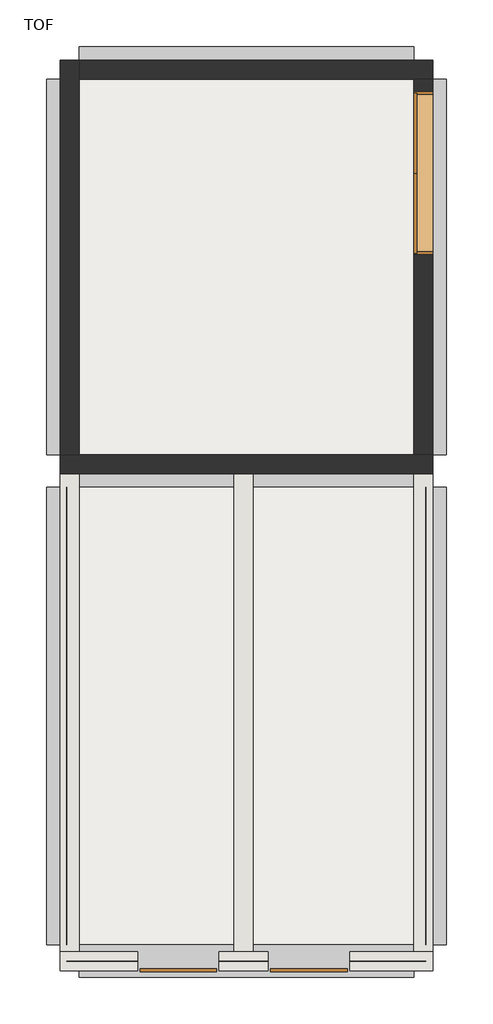
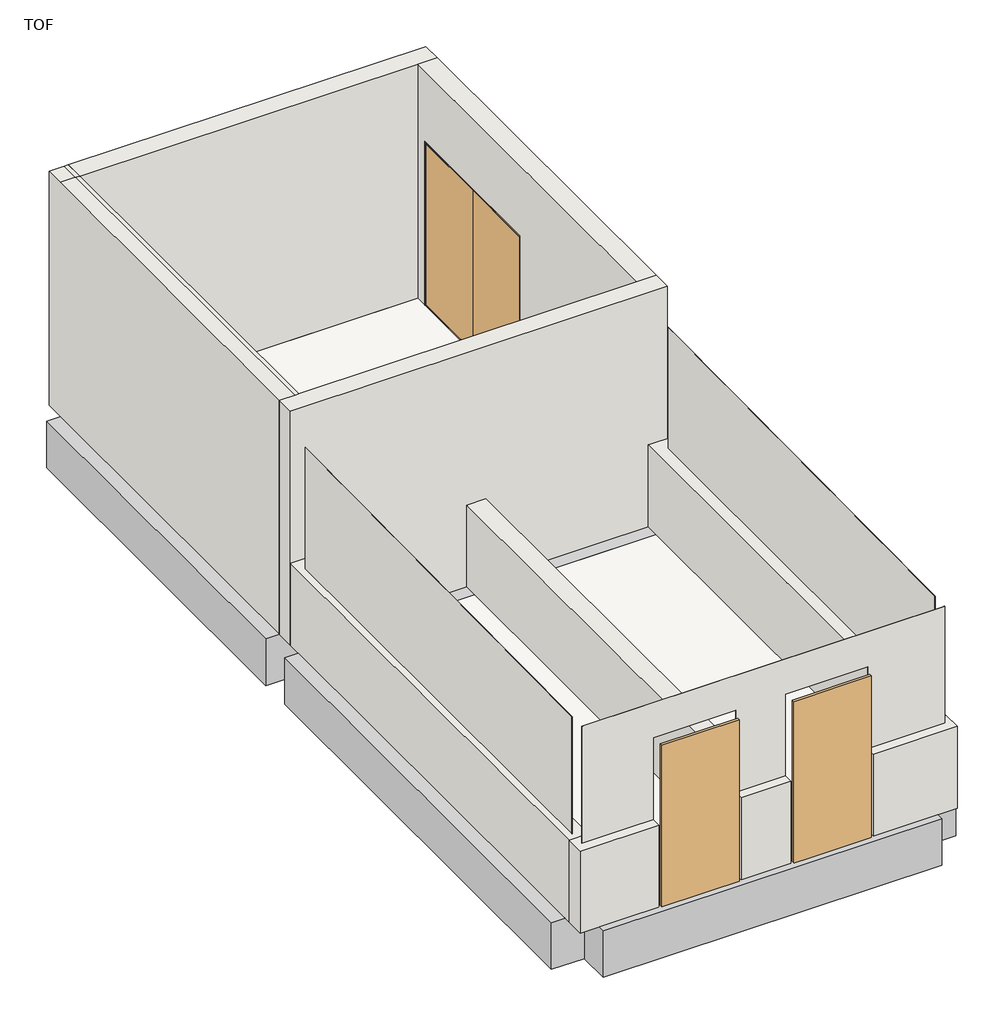
# One storey: 11 walls, 7 beams, 3 doors, 2 slabs.
"""IFC4 building model written with IfcOpenShell, lengths in millimetres."""

import ifcopenshell
import ifcopenshell.guid

model = None  # the IFC model being written
_history = None  # IfcOwnerHistory: only IFC2X3 demands one
_inside = {}  # id of a spatial element -> (the spatial element, [elements in it])
_under = {}  # id of a project, library or spatial element -> (it, [spatial elements below it])
_declared = {}  # id of a project -> (the project, [libraries it declares])
_typed = {}  # id of a type object -> (the type object, [elements of that type])
_made_of = {}  # id of a material, layer set ... -> (it, [elements and type objects made of it])


def new_model(schema):
    """Start an empty IFC model of exactly this schema.

    Asked for "IFC4X3", IfcOpenShell would pick the latest addendum, in which some entities
    have other attributes; the version numbers below select the first issue.
    IFC2X3 requires an IfcOwnerHistory on every rooted entity: one is made here for all.
    """
    global model, _history
    if schema == "IFC4X3":
        model = ifcopenshell.file(schema_version=(4, 3, 0, 0))
    else:
        model = ifcopenshell.file(schema=schema)
    _inside.clear()
    _under.clear()
    _declared.clear()
    _typed.clear()
    _made_of.clear()
    _history = None
    if model.schema == "IFC2X3":
        org = make("IfcOrganization", Name="unknown")
        user = make(
            "IfcPersonAndOrganization",
            ThePerson=make("IfcPerson", FamilyName="unknown"),
            TheOrganization=org,
        )
        app = make(
            "IfcApplication",
            ApplicationDeveloper=org,
            Version="unknown",
            ApplicationFullName="unknown",
            ApplicationIdentifier="unknown",
        )
        _history = make(
            "IfcOwnerHistory",
            OwningUser=user,
            OwningApplication=app,
            ChangeAction="ADDED",
            CreationDate=0,
        )
    return model


def make(cls, **values):
    """One entity of the class cls with the attributes given. An attribute that is None is left unset."""
    return model.create_entity(
        cls, **{name: value for name, value in values.items() if value is not None}
    )


def rooted(cls, **values):
    """An entity with a GlobalId (a new one), such as an element, a storey or a relation."""
    return make(cls, GlobalId=ifcopenshell.guid.new(), OwnerHistory=_history, **values)


def si_unit(unit_type, name, prefix=None):
    """IfcSIUnit, for example si_unit("LENGTHUNIT", "METRE", prefix="MILLI")."""
    return make("IfcSIUnit", UnitType=unit_type, Prefix=prefix, Name=name)


def assignment(units):
    """IfcUnitAssignment: the units of a project."""
    return None if units is None else make("IfcUnitAssignment", Units=units)


def point(xyz):
    """IfcCartesianPoint."""
    return None if xyz is None else make("IfcCartesianPoint", Coordinates=xyz)


def direction(xyz):
    """IfcDirection."""
    return None if xyz is None else make("IfcDirection", DirectionRatios=xyz)


def frame(location, z_axis=None, x_axis=None):
    """IfcAxis2Placement3D, a coordinate frame: its origin and axes. An axis left out is left unset."""
    return make(
        "IfcAxis2Placement3D",
        Location=point(location),
        Axis=direction(z_axis),
        RefDirection=direction(x_axis),
    )


def origin():
    """The frame at (0, 0, 0) with its axes left unset."""
    return frame((0.0, 0.0, 0.0))


def origin_with_axes():
    """The frame at (0, 0, 0) with the z axis (0, 0, 1) and the x axis (1, 0, 0) written out."""
    return frame((0.0, 0.0, 0.0), z_axis=(0.0, 0.0, 1.0), x_axis=(1.0, 0.0, 0.0))


def place(relative_to, where):
    """IfcLocalPlacement: puts the frame where relative to a parent placement (None: the world)."""
    return make(
        "IfcLocalPlacement", PlacementRelTo=relative_to, RelativePlacement=where
    )


def context(
    kind, dimensions, precision=None, world=None, true_north=None, identifier=None
):
    """IfcGeometricRepresentationContext, for example the 3D "Model" context."""
    return make(
        "IfcGeometricRepresentationContext",
        ContextIdentifier=identifier,
        ContextType=kind,
        CoordinateSpaceDimension=dimensions,
        Precision=precision,
        WorldCoordinateSystem=world,
        TrueNorth=true_north,
    )


def project(units=None, contexts=None):
    """IfcProject with its units and contexts."""
    return rooted(
        "IfcProject",
        Name="project",
        RepresentationContexts=contexts,
        UnitsInContext=assignment(units),
    )


def spatial(cls, under=None, at=None, **own):
    """A site, building, storey or space (cls), placed at a placement, below another one or the project."""
    s = rooted(cls, ObjectPlacement=at, **own)
    if under is not None:
        _under.setdefault(under.id(), (under, []))[1].append(s)
    return s


def polyline(points):
    """IfcPolyline through the points."""
    return make("IfcPolyline", Points=[point(p) for p in points])


def outline(outer, holes=None, kind="AREA"):
    """IfcArbitraryClosedProfileDef: a profile drawn as a closed curve; with holes, ...WithVoids."""
    if holes is None:
        return make("IfcArbitraryClosedProfileDef", ProfileType=kind, OuterCurve=outer)
    return make(
        "IfcArbitraryProfileDefWithVoids",
        ProfileType=kind,
        OuterCurve=outer,
        InnerCurves=holes,
    )


def extrude(swept, where, along, depth):
    """IfcExtrudedAreaSolid: the profile swept, set in the frame where, extruded along a direction by depth."""
    return make(
        "IfcExtrudedAreaSolid",
        SweptArea=swept,
        Position=where,
        ExtrudedDirection=direction(along),
        Depth=depth,
    )


def faces_of(points, faces, orient=None, outer=None):
    """IfcFace entities. A face is a list of loops; a loop is a list of indices into points, from 0.

    orient and outer hold one flag for each loop. By default every Orientation is true, the
    first loop of a face is its IfcFaceOuterBound and the others are IfcFaceBound.
    """
    made = []
    for i, loops in enumerate(faces):
        bounds = []
        for j, loop in enumerate(loops):
            is_outer = j == 0 if outer is None else outer[i][j]
            bounds.append(
                make(
                    "IfcFaceOuterBound" if is_outer else "IfcFaceBound",
                    Bound=make("IfcPolyLoop", Polygon=[points[k] for k in loop]),
                    Orientation=True if orient is None else orient[i][j],
                )
            )
        made.append(make("IfcFace", Bounds=bounds))
    return made


def faceted_brep(points, faces, orient=None, outer=None, voids=None):
    """IfcFacetedBrep: a solid bounded by flat faces; with voids (closed shells), ...WithVoids."""
    shared = [point(p) for p in points]
    hull = make("IfcClosedShell", CfsFaces=faces_of(shared, faces, orient, outer))
    if voids is None:
        return make("IfcFacetedBrep", Outer=hull)
    return make(
        "IfcFacetedBrepWithVoids",
        Outer=hull,
        Voids=[
            make(cls, CfsFaces=faces_of(shared, fs, o, b)) for cls, fs, o, b in voids
        ],
    )


def shape(context_of_items, identifier, shape_type, items):
    """IfcShapeRepresentation: the items that make up one representation, for example the "Body"."""
    return make(
        "IfcShapeRepresentation",
        ContextOfItems=context_of_items,
        RepresentationIdentifier=identifier,
        RepresentationType=shape_type,
        Items=items,
    )


def source(mapping_origin, context_of_items, identifier, shape_type, items):
    """IfcRepresentationMap: a shape defined once, which mapped items show again and again."""
    return make(
        "IfcRepresentationMap",
        MappingOrigin=mapping_origin,
        MappedRepresentation=shape(context_of_items, identifier, shape_type, items),
    )


def transform(
    local_origin,
    x_axis=None,
    y_axis=None,
    z_axis=None,
    scale=None,
    scale2=None,
    scale3=None,
    uniform=True,
):
    """IfcCartesianTransformationOperator3D, or its non-uniform kind. x_axis, y_axis, z_axis: its Axis1, 2, 3."""
    if uniform:
        return make(
            "IfcCartesianTransformationOperator3D",
            Axis1=direction(x_axis),
            Axis2=direction(y_axis),
            LocalOrigin=point(local_origin),
            Scale=scale,
            Axis3=direction(z_axis),
        )
    return make(
        "IfcCartesianTransformationOperator3DnonUniform",
        Axis1=direction(x_axis),
        Axis2=direction(y_axis),
        LocalOrigin=point(local_origin),
        Scale=scale,
        Axis3=direction(z_axis),
        Scale2=scale2,
        Scale3=scale3,
    )


def mapped(mapping_source, mapping_target):
    """IfcMappedItem: shows the shape of a source again, moved by a transform."""
    return make(
        "IfcMappedItem", MappingSource=mapping_source, MappingTarget=mapping_target
    )


def made_of(thing, what):
    """Note that an element or type object is made of a material, layer set ...; save() writes the relation."""
    if what is not None:
        _made_of.setdefault(what.id(), (what, []))[1].append(thing)
    return thing


def element(
    cls,
    number,
    at=None,
    inside=None,
    cuts=None,
    type_object=None,
    material=None,
    context=None,
    identifier="Body",
    shape_type=None,
    held_by="IfcProductDefinitionShape",
    body=None,
    shapes=None,
    **own,
):
    """One element of the class cls, such as IfcWall. Its Tag is "e" and its number.

    at: its placement. inside: the storey or other place that contains it. cuts: it is an
    opening in that element (IfcRelVoidsElement). A single representation is given by context,
    identifier, shape_type and body (its items); several are given by shapes. held_by: the class
    of the entity that holds the representations. save() writes the other relations.
    """
    e = rooted(cls, Tag="e%d" % number, ObjectPlacement=at, **own)
    if body is not None:
        shapes = [shape(context, identifier, shape_type, body)]
    if shapes is not None:
        e.Representation = make(held_by, Representations=shapes)
    if inside is not None:
        _inside.setdefault(inside.id(), (inside, []))[1].append(e)
    if cuts is not None:
        rooted(
            "IfcRelVoidsElement", RelatingBuildingElement=cuts, RelatedOpeningElement=e
        )
    if type_object is not None:
        _typed.setdefault(type_object.id(), (type_object, []))[1].append(e)
    return made_of(e, material)


def aggregate(whole, parts):
    """IfcRelAggregates: a whole, such as a stair, and the parts it consists of."""
    return rooted("IfcRelAggregates", RelatingObject=whole, RelatedObjects=parts)


def save(model, path):
    """Write the relations noted so far, then the file.

    IfcRelAggregates (storeys below a building ...), IfcRelContainedInSpatialStructure (elements
    in a storey), IfcRelDefinesByType, IfcRelAssociatesMaterial and IfcRelDeclares: one each for
    every whole, place, type object, material and project.
    """
    for whole, parts in _under.values():
        aggregate(whole, parts)
    for where, things in _inside.values():
        rooted(
            "IfcRelContainedInSpatialStructure",
            RelatedElements=things,
            RelatingStructure=where,
        )
    for kind, things in _typed.values():
        rooted("IfcRelDefinesByType", RelatedObjects=things, RelatingType=kind)
    for what, things in _made_of.values():
        rooted("IfcRelAssociatesMaterial", RelatedObjects=things, RelatingMaterial=what)
    for by, libraries in _declared.values():
        rooted("IfcRelDeclares", RelatingContext=by, RelatedDefinitions=libraries)
    model.write(path)


def double_door_steel_cbf312ec(model_context):
    return source(origin(), model_context, "Body", "SolidModel", [
        extrude(outline(polyline([(980.0, 77.0), (0.0, 77.0), (0.0, 117.0), (980.0, 117.0), (980.0, 77.0)])), frame((0.0, 0.0, 20.0), z_axis=(0.0, 0.0, 1.0), x_axis=(1.0, 0.0, 0.0)), (0.0, 0.0, 1.0), 2060.0),
        extrude(outline(polyline([(0.0, 77.0), (-980.0, 77.0), (-980.0, 117.0), (0.0, 117.0), (0.0, 77.0)])), frame((0.0, 0.0, 20.0), z_axis=(0.0, 0.0, 1.0), x_axis=(1.0, 0.0, 0.0)), (0.0, 0.0, 1.0), 2060.0),
        faceted_brep([(1000.0, -117.0, 2100.0), (1000.0, 117.0, 2100.0), (-1000.0, 117.0, 2100.0), (-1000.0, -117.0, 2100.0), (965.0, 77.0, 2065.0), (965.0, -117.0, 2065.0), (-965.0, -117.0, 2065.0), (-965.0, 77.0, 2065.0), (980.0, 117.0, 2080.0), (980.0, 77.0, 2080.0), (-980.0, 77.0, 2080.0), (-980.0, 117.0, 2080.0), (-1000.0, 117.0, 0.0), (-1000.0, -117.0, 0.0), (-965.0, -117.0, 35.0), (-965.0, 77.0, 35.0), (-980.0, 77.0, 20.0), (-980.0, 117.0, 20.0), (1000.0, 117.0, 0.0), (980.0, 117.0, 20.0), (1000.0, -117.0, 0.0), (965.0, -117.0, 35.0), (965.0, 77.0, 35.0), (980.0, 77.0, 20.0)], [[[0, 1, 2, 3]], [[4, 5, 6, 7]], [[8, 9, 10, 11]], [[3, 2, 12, 13]], [[7, 6, 14, 15]], [[11, 10, 16, 17]], [[18, 12, 2, 1], [8, 11, 17, 19]], [[13, 12, 18, 20]], [[0, 3, 13, 20], [21, 14, 6, 5]], [[15, 14, 21, 22]], [[23, 16, 10, 9], [4, 7, 15, 22]], [[17, 16, 23, 19]], [[20, 18, 1, 0]], [[22, 21, 5, 4]], [[19, 23, 9, 8]]]),
    ])


def single_door_steel_bf6f5e52(model_context):
    return source(origin(), model_context, "Body", "SweptSolid", [
        extrude(outline(polyline([(470.0, -130.0), (-470.0, -130.0), (-470.0, -95.0), (470.0, -95.0), (470.0, -130.0)])), origin_with_axes(), (0.0, 0.0, 1.0), 2070.0),
    ])


model = new_model("IFC4")

# Units and contexts
model_context = context("Model", 3, world=origin())
ifc_project = project(units=[si_unit("LENGTHUNIT", "METRE", prefix="MILLI")], contexts=[model_context])

# Site, building, storey
site = spatial("IfcSite", under=ifc_project)
building = spatial("IfcBuilding", under=site)
storey = spatial("IfcBuildingStorey", under=building, Name="TOF", Elevation=200250.0)

# Beams
placement = place(None, origin())
element("IfcBeam", 1, ObjectType="RC Beam_Rectangular : H_SB_ACB_TG_B500xH500", at=placement, inside=storey, context=model_context, shape_type="Brep", body=[
    faceted_brep([(-1563.0, -1039.9791411, 200250.0), (-1963.0, -1039.9791411, 200250.0), (-1963.0, -1039.9791411, 199650.0), (-1563.0, -1039.9791411, 199650.0), (-1563.0, -1039.9791411, 200100.0), (-1963.0, 4560.0208589, 200250.0), (-1563.0, 4560.0208589, 200250.0), (-1563.0, 4560.0208589, 200100.0), (-1563.0, 4560.0208589, 199650.0), (-1963.0, 4560.0208589, 199650.0)], [[[0, 1, 2, 3, 4]], [[5, 6, 7, 8, 9]], [[1, 0, 6, 5]], [[2, 1, 5, 9]], [[3, 2, 9, 8]], [[0, 4, 3, 8, 7, 6]]]),
])
element("IfcBeam", 2, ObjectType="RC Beam_Rectangular : H_SB_ACB_TG_B500xH500", at=placement, inside=storey, context=model_context, shape_type="Brep", body=[
    faceted_brep([(-1563.0, -1439.9791411, 200250.0), (-1563.0, -1039.9791411, 200250.0), (-1563.0, -1039.9791411, 200100.0), (-1563.0, -1039.9791411, 199650.0), (-1563.0, -1439.9791411, 199650.0), (2537.0, -1039.9791411, 200250.0), (2537.0, -1439.9791411, 200250.0), (2537.0, -1439.9791411, 199650.0), (2537.0, -1039.9791411, 199650.0), (2537.0, -1039.9791411, 200100.0)], [[[0, 1, 2, 3, 4]], [[5, 6, 7, 8, 9]], [[1, 0, 6, 5]], [[0, 4, 7, 6]], [[4, 3, 8, 7]], [[3, 2, 1, 5, 9, 8]]]),
])
element("IfcBeam", 3, ObjectType="RC Beam_Rectangular : H_SB_ACB_TG_B500xH500", at=placement, inside=storey, context=model_context, shape_type="Brep", body=[
    faceted_brep([(-1563.0, 4560.0208589, 200250.0), (-1563.0, 4960.0208589, 200250.0), (-1563.0, 4960.0208589, 200100.0), (-1563.0, 4960.0208589, 199650.0), (-1563.0, 4560.0208589, 199650.0), (-1563.0, 4560.0208589, 200100.0), (2537.0, 4960.0208589, 200250.0), (2537.0, 4560.0208589, 200250.0), (2537.0, 4560.0208589, 200100.0), (2537.0, 4560.0208589, 199650.0), (2537.0, 4960.0208589, 199650.0), (2537.0, 4960.0208589, 200100.0)], [[[0, 1, 2, 3, 4, 5]], [[6, 7, 8, 9, 10, 11]], [[1, 0, 7, 6]], [[0, 5, 4, 9, 8, 7]], [[4, 3, 10, 9]], [[3, 2, 1, 6, 11, 10]]]),
])
element("IfcBeam", 4, ObjectType="RC Beam_Rectangular : H_SB_ACB_TG_B500xH500", at=placement, inside=storey, context=model_context, shape_type="Brep", body=[
    faceted_brep([(2937.0, 4560.0208589, 200250.0), (2537.0, 4560.0208589, 200250.0), (2537.0, -1039.9791411, 200250.0), (2937.0, -1039.9791411, 200250.0), (2537.0, -1039.9791411, 199650.0), (2537.0, -1039.9791411, 200100.0), (2537.0, 4560.0208589, 200100.0), (2537.0, 4560.0208589, 199650.0), (2937.0, 4560.0208589, 199650.0), (2937.0, -1039.9791411, 199650.0)], [[[0, 1, 2, 3]], [[4, 5, 2, 1, 6, 7]], [[7, 8, 9, 4]], [[3, 9, 8, 0]], [[2, 5, 4, 9, 3]], [[7, 6, 1, 0, 8]]]),
])
element("IfcBeam", 5, ObjectType="RC Beam_Rectangular : H_SB_ACB_TG_B500xH500", at=placement, inside=storey, context=model_context, shape_type="Brep", body=[
    faceted_brep([(-1963.0, 9560.0208589, 200250.0), (-1563.0, 9560.0208589, 200250.0), (-1563.0, 9560.0208589, 200100.0), (-1563.0, 9560.0208589, 199650.0), (-1963.0, 9560.0208589, 199650.0), (-1563.0, 4960.0208589, 200250.0), (-1963.0, 4960.0208589, 200250.0), (-1963.0, 4960.0208589, 199650.0), (-1563.0, 4960.0208589, 199650.0), (-1563.0, 4960.0208589, 200100.0)], [[[0, 1, 2, 3, 4]], [[5, 6, 7, 8, 9]], [[1, 0, 6, 5]], [[0, 4, 7, 6]], [[4, 3, 8, 7]], [[3, 2, 1, 5, 9, 8]]]),
])
element("IfcBeam", 6, ObjectType="RC Beam_Rectangular : H_SB_ACB_TG_B400xH600", at=placement, inside=storey, context=model_context, shape_type="Brep", body=[
    faceted_brep([(-1563.0, 9960.0208589, 200250.0), (-1563.0, 9560.0208589, 200250.0), (2537.0, 9560.0208589, 200250.0), (2537.0, 9960.0208589, 200250.0), (-1563.0, 9560.0208589, 200100.0), (-1563.0, 9560.0208589, 199650.0), (2537.0, 9560.0208589, 199650.0), (2537.0, 9560.0208589, 200100.0), (-1563.0, 9960.0208589, 199650.0), (2537.0, 9960.0208589, 199650.0)], [[[0, 1, 2, 3]], [[1, 4, 5, 6, 7, 2]], [[5, 8, 9, 6]], [[8, 0, 3, 9]], [[1, 0, 8, 5, 4]], [[3, 2, 7, 6, 9]]]),
])
element("IfcBeam", 7, ObjectType="RC Beam_Rectangular : H_SB_ACB_TG_B500xH500", at=placement, inside=storey, context=model_context, shape_type="Brep", body=[
    faceted_brep([(2937.0, 4960.0208589, 200250.0), (2537.0, 4960.0208589, 200250.0), (2537.0, 4960.0208589, 200100.0), (2537.0, 4960.0208589, 199650.0), (2937.0, 4960.0208589, 199650.0), (2937.0, 9560.0208589, 200250.0), (2537.0, 9560.0208589, 200250.0), (2537.0, 9560.0208589, 200100.0), (2537.0, 9560.0208589, 199650.0), (2937.0, 9560.0208589, 199650.0)], [[[0, 1, 2, 3, 4]], [[1, 0, 5, 6]], [[1, 6, 7, 8, 3, 2]], [[4, 3, 8, 9]], [[0, 4, 9, 5]], [[5, 9, 8, 7, 6]]]),
])

# Doors
double_door_steel_shape = double_door_steel_cbf312ec(model_context)
element("IfcDoor", 8, ObjectType="Double Door_Steel : H_DR_AMB_Double Door_Steel_W2000xH2100", at=placement, inside=storey, context=model_context, shape_type="MappedRepresentation", body=[
    mapped(double_door_steel_shape, transform((2654.0, 8410.0208589, 200250.0), x_axis=(0.0, 1.0, 0.0), y_axis=(-1.0, 0.0, 0.0), z_axis=(0.0, 0.0, 1.0))),
])
single_door_steel_shape = single_door_steel_bf6f5e52(model_context)
element("IfcDoor", 9, ObjectType="Single Door_Steel : H_DR_AMB_Single Door_Steel_W1000xH2100", at=placement, inside=storey, context=model_context, shape_type="MappedRepresentation", body=[
    mapped(single_door_steel_shape, transform((-346.0, -1239.9791411, 200250.0), x_axis=(1.0, 0.0, 0.0), y_axis=(0.0, 1.0, 0.0), z_axis=(0.0, 0.0, 1.0))),
])
element("IfcDoor", 10, ObjectType="Single Door_Steel : H_DR_AMB_Single Door_Steel_W1000xH2100", at=placement, inside=storey, context=model_context, shape_type="MappedRepresentation", body=[
    mapped(single_door_steel_shape, transform((1254.0, -1239.9791411, 200250.0), x_axis=(1.0, 0.0, 0.0), y_axis=(0.0, 1.0, 0.0), z_axis=(0.0, 0.0, 1.0))),
])

# Slabs
element("IfcSlab", 11, ObjectType="H_SF_ACF_SOG T150", at=placement, inside=storey, context=model_context, shape_type="SweptSolid", body=[
    extrude(outline(polyline([(2537.0, 9560.0208589), (2537.0, 4960.0208589), (-1563.0, 4960.0208589), (-1563.0, 9560.0208589), (2537.0, 9560.0208589)])), frame((0.0, 0.0, 200100.0), z_axis=(0.0, 0.0, 1.0), x_axis=(1.0, 0.0, 0.0)), (0.0, 0.0, 1.0), 150.0),
])
element("IfcSlab", 12, ObjectType="H_SF_ACF_SOG T150", at=placement, inside=storey, context=model_context, shape_type="SweptSolid", body=[
    extrude(outline(polyline([(2537.0, 4560.0208589), (2537.0, -1039.9791411), (-1563.0, -1039.9791411), (-1563.0, 4560.0208589), (2537.0, 4560.0208589)])), frame((0.0, 0.0, 200100.0), z_axis=(0.0, 0.0, 1.0), x_axis=(1.0, 0.0, 0.0)), (0.0, 0.0, 1.0), 150.0),
])

# Walls
element("IfcWall", 13, ObjectType="H_WA_AMW_Block Wall_Int_T200 (Both Plaster_Emulsion)", at=placement, inside=storey, context=model_context, shape_type="Brep", body=[
    faceted_brep([(-1797.0, 9794.0208589, 200250.0), (-1797.0, 4960.0208589, 200250.0), (-1797.0, 4960.0208589, 203250.0), (-1797.0, 9560.0208589, 203250.0), (-1797.0, 9794.0208589, 203250.0), (-1563.0, 9794.0208589, 200250.0), (-1563.0, 9794.0208589, 203250.0), (-1563.0, 9560.0208589, 203250.0), (-1563.0, 4960.0208589, 203250.0), (-1563.0, 4960.0208589, 200250.0), (-1563.0, 9560.0208589, 200250.0), (-1613.0, 9794.0208589, 203250.0), (-1613.0, 4960.0208589, 203250.0), (-1613.0, 9560.0208589, 203250.0)], [[[0, 1, 2, 3, 4]], [[5, 6, 7, 8, 9, 10]], [[1, 0, 5, 10, 9]], [[0, 4, 11, 6, 5]], [[1, 9, 8, 12, 2]], [[7, 6, 11, 13]], [[3, 2, 12, 13]], [[4, 3, 13, 11]], [[12, 8, 7, 13]]]),
])
element("IfcWall", 14, ObjectType="H_WA_AMW_Block Wall_Int_T200 (Both Plaster_Emulsion)", at=placement, inside=storey, context=model_context, shape_type="Brep", body=[
    faceted_brep([(-1797.0, 4726.0208589, 203250.0), (-1797.0, 4726.0208589, 201300.0), (-1797.0, 4726.0208589, 200250.0), (-1563.0, 4726.0208589, 200250.0), (337.0, 4726.0208589, 200250.0), (571.0, 4726.0208589, 200250.0), (2537.0, 4726.0208589, 200250.0), (2771.0, 4726.0208589, 200250.0), (2771.0, 4726.0208589, 201300.0), (2771.0, 4726.0208589, 203250.0), (-1797.0, 4960.0208589, 200250.0), (-1797.0, 4960.0208589, 203250.0), (-1563.0, 4960.0208589, 203250.0), (2537.0, 4960.0208589, 203250.0), (2771.0, 4960.0208589, 203250.0), (2771.0, 4960.0208589, 200250.0), (2537.0, 4960.0208589, 200250.0), (-1563.0, 4960.0208589, 200250.0)], [[[0, 1, 2, 3, 4, 5, 6, 7, 8, 9]], [[10, 11, 12, 13, 14, 15, 16, 17]], [[7, 6, 5, 4, 3, 2, 10, 17, 16, 15]], [[0, 9, 14, 13, 12, 11]], [[7, 15, 14, 9, 8]], [[0, 11, 10, 2, 1]]]),
])
element("IfcWall", 15, ObjectType="H_WA_AMW_Block Wall_Int_T200 (Both Plaster_Emulsion)", at=placement, inside=storey, context=model_context, shape_type="SweptSolid", body=[
    extrude(outline(polyline([(2771.0, 4726.0208589), (2771.0, -1122.9791411), (2537.0, -1122.9791411), (2537.0, 4726.0208589), (2771.0, 4726.0208589)])), frame((0.0, 0.0, 200250.0), z_axis=(0.0, 0.0, 1.0), x_axis=(1.0, 0.0, 0.0)), (0.0, 0.0, 1.0), 1050.0),
])
element("IfcWall", 16, ObjectType="H_WA_AMW_Block Wall_Int_T200 (Both Plaster_Emulsion)", at=placement, inside=storey, context=model_context, shape_type="Brep", body=[
    faceted_brep([(2771.0, 9794.0208589, 200250.0), (-1563.0, 9794.0208589, 200250.0), (-1563.0, 9794.0208589, 203250.0), (2771.0, 9794.0208589, 203250.0), (2771.0, 9560.0208589, 200250.0), (2771.0, 9560.0208589, 203250.0), (2537.0, 9560.0208589, 203250.0), (-1563.0, 9560.0208589, 203250.0), (-1563.0, 9560.0208589, 200250.0), (2537.0, 9560.0208589, 200250.0)], [[[0, 1, 2, 3]], [[4, 5, 6, 7, 8, 9]], [[1, 0, 4, 9, 8]], [[3, 2, 7, 6, 5]], [[2, 1, 8, 7]], [[0, 3, 5, 4]]]),
])
element("IfcWall", 17, ObjectType="H_WA_AMW_Block Wall_Int_T200 (Both Plaster_Emulsion)", at=placement, inside=storey, context=model_context, shape_type="Brep", body=[
    faceted_brep([(2771.0, -1356.9791411, 200250.0), (2771.0, -1356.9791411, 201300.0), (1754.0, -1356.9791411, 201300.0), (1754.0, -1356.9791411, 200250.0), (2771.0, -1122.9791411, 201300.0), (2771.0, -1122.9791411, 200250.0), (2537.0, -1122.9791411, 200250.0), (1754.0, -1122.9791411, 200250.0), (1754.0, -1122.9791411, 201300.0), (2537.0, -1122.9791411, 201300.0)], [[[0, 1, 2, 3]], [[4, 5, 6, 7, 8, 9]], [[5, 0, 3, 7, 6]], [[1, 4, 9, 8, 2]], [[1, 0, 5, 4]], [[3, 2, 8, 7]]]),
    faceted_brep([(-1797.0, -1356.9791411, 201300.0), (-1797.0, -1356.9791411, 200250.0), (-846.0, -1356.9791411, 200250.0), (-846.0, -1356.9791411, 201300.0), (-1797.0, -1122.9791411, 200250.0), (-1797.0, -1122.9791411, 201300.0), (-1563.0, -1122.9791411, 201300.0), (-846.0, -1122.9791411, 201300.0), (-846.0, -1122.9791411, 200250.0), (-1563.0, -1122.9791411, 200250.0)], [[[0, 1, 2, 3]], [[4, 5, 6, 7, 8, 9]], [[1, 4, 9, 8, 2]], [[5, 0, 3, 7, 6]], [[1, 0, 5, 4]], [[3, 2, 8, 7]]]),
    faceted_brep([(154.0, -1356.9791411, 201300.0), (154.0, -1356.9791411, 200250.0), (754.0, -1356.9791411, 200250.0), (754.0, -1356.9791411, 201300.0), (154.0, -1122.9791411, 200250.0), (154.0, -1122.9791411, 201300.0), (337.0, -1122.9791411, 201300.0), (571.0, -1122.9791411, 201300.0), (754.0, -1122.9791411, 201300.0), (754.0, -1122.9791411, 200250.0), (571.0, -1122.9791411, 200250.0), (337.0, -1122.9791411, 200250.0)], [[[0, 1, 2, 3]], [[4, 5, 6, 7, 8, 9, 10, 11]], [[1, 4, 11, 10, 9, 2]], [[5, 0, 3, 8, 7, 6]], [[1, 0, 5, 4]], [[3, 2, 9, 8]]]),
])
element("IfcWall", 18, ObjectType="H_WA_AMW_Block Wall_Int_T200 (Both Plaster_Emulsion)", at=placement, inside=storey, context=model_context, shape_type="SweptSolid", body=[
    extrude(outline(polyline([(4960.0208589, 203250.0), (9560.0208589, 203250.0), (9560.0208589, 200250.0), (9410.0208589, 200250.0), (9410.0208589, 202350.0), (7410.0208589, 202350.0), (7410.0208589, 200250.0), (4960.0208589, 200250.0), (4960.0208589, 203250.0)])), frame((2537.0, 0.0, 0.0), z_axis=(1.0, 0.0, 0.0), x_axis=(0.0, 1.0, 0.0)), (0.0, 0.0, 1.0), 234.0),
])
element("IfcWall", 19, ObjectType="H_WA_AMW_Block Wall_Int_T200 (Both Plaster_Emulsion)", at=placement, inside=storey, context=model_context, shape_type="SweptSolid", body=[
    extrude(outline(polyline([(-1563.0, 4726.0208589), (-1563.0, -1122.9791411), (-1797.0, -1122.9791411), (-1797.0, 4726.0208589), (-1563.0, 4726.0208589)])), frame((0.0, 0.0, 200250.0), z_axis=(0.0, 0.0, 1.0), x_axis=(1.0, 0.0, 0.0)), (0.0, 0.0, 1.0), 1050.0),
])
element("IfcWall", 20, ObjectType="H_WA_AMW_Wall Single Sheet_T0.7", at=placement, inside=storey, context=model_context, shape_type="SweptSolid", body=[
    extrude(outline(polyline([(201300.0, 2687.0), (202800.0, 2687.0), (202800.0, -1713.0), (201300.0, -1713.0), (201300.0, -846.0), (202350.0, -846.0), (202350.0, 154.0), (201300.0, 154.0), (201300.0, 754.0), (202350.0, 754.0), (202350.0, 1754.0), (201300.0, 1754.0), (201300.0, 2687.0)])), frame((0.0, -1240.4791411, 0.0), z_axis=(0.0, 1.0, 0.0), x_axis=(0.0, 0.0, 1.0)), (0.0, 0.0, 1.0), 1.0),
])
element("IfcWall", 21, ObjectType="H_WA_AMW_Wall Single Sheet_T0.7", at=placement, inside=storey, context=model_context, shape_type="SweptSolid", body=[
    extrude(outline(polyline([(-1039.9791411, 201300.0), (-1039.9791411, 202802.5), (4560.0208589, 202857.5), (4560.0208589, 201300.0), (-1039.9791411, 201300.0)])), frame((-1714.0, 0.0, 0.0), z_axis=(1.0, 0.0, 0.0), x_axis=(0.0, 1.0, 0.0)), (0.0, 0.0, 1.0), 1.0),
])
element("IfcWall", 22, ObjectType="H_WA_AMW_Block Wall_Int_T200 (Both Plaster_Emulsion)", at=placement, inside=storey, context=model_context, shape_type="SweptSolid", body=[
    extrude(outline(polyline([(571.0, 4726.0208589), (571.0, -1122.9791411), (337.0, -1122.9791411), (337.0, 4726.0208589), (571.0, 4726.0208589)])), frame((0.0, 0.0, 200250.0), z_axis=(0.0, 0.0, 1.0), x_axis=(1.0, 0.0, 0.0)), (0.0, 0.0, 1.0), 1050.0),
])
element("IfcWall", 23, ObjectType="H_WA_AMW_Wall Single Sheet_T0.7", at=placement, inside=storey, context=model_context, shape_type="SweptSolid", body=[
    extrude(outline(polyline([(-1039.9791411, 201300.0), (-1039.9791411, 202802.5), (4560.0208589, 202857.5), (4560.0208589, 201300.0), (-1039.9791411, 201300.0)])), frame((2686.0, 0.0, 0.0), z_axis=(1.0, 0.0, 0.0), x_axis=(0.0, 1.0, 0.0)), (0.0, 0.0, 1.0), 1.0),
])

save(model, "model.ifc")

# Revit data of these elements
# Project information
#   Building Name = "SULFUR LOADING CONTROL BD"
#   Project Status = "Project Status"
#   Client Name = "현대엔지니어링"
#   Project Address = "서울시 종로구 율곡로 75(계동)"
#   Project Number = "-"
# Grids (mm)
#   "1": line (-1763, 13601.905) -> (-1763, -6521.949)
#   "2": line (2737, 13601.905) -> (2737, -6521.949)
#   "B": line (-5623.098, 4760.021) -> (9120.042, 4760.021)
#   "A": line (-5623.098, -1239.979) -> (9120.042, -1239.979)
#   "C": line (-5623.098, 9760.021) -> (9120.042, 9760.021)
# Type "RC Beam_Rectangular : H_SB_ACB_TG_B500xH500"
#   중앙부 하부근 = ""
#   중앙부 상부근 = ""
#   중앙부 보조근 = ""
#   중앙부 늑근 = ""
#   외단부 하부근 = ""
#   외단부 상부근 = ""
#   외단부 보조근 = ""
#   외단부 늑근 = ""
#   부호 = "TG2"
#   내단부 하부근 = ""
#   내단부 상부근 = ""
#   내단부 보조근 = ""
#   내단부 늑근 = ""
#   ALL 하부근 = "3-D20"
#   ALL 상부근 = "4-D20"
#   ALL 보조근 = ""
#   ALL 늑근 = "2-D10 @120"
#   Width = 400.000 mm
#   Height = 600.000 mm
#   Length [instance default] = 1524.000 mm
#   b = 400.000 mm
#   h = 600.000 mm
#   hec_material3 [instance default] = none
#   hec_material2 [instance default] = none
#   hec_material1 [instance default] = none
#   Structural Material [instance default] = none
#   Assembly Code = ""
# Type "RC Beam_Rectangular : H_SB_ACB_TG_B400xH600"
#   중앙부 하부근 = ""
#   중앙부 상부근 = ""
#   중앙부 보조근 = ""
#   중앙부 늑근 = ""
#   외단부 하부근 = ""
#   외단부 상부근 = ""
#   외단부 보조근 = ""
#   외단부 늑근 = ""
#   부호 = "TG2"
#   내단부 하부근 = ""
#   내단부 상부근 = ""
#   내단부 보조근 = ""
#   내단부 늑근 = ""
#   ALL 하부근 = "3-D20"
#   ALL 상부근 = "4-D20"
#   ALL 보조근 = ""
#   ALL 늑근 = "2-D10 @120"
#   Width = 400.000 mm
#   Height = 600.000 mm
#   Length [instance default] = 1524.000 mm
#   b = 400.000 mm
#   h = 600.000 mm
#   hec_material3 [instance default] = none
#   hec_material2 [instance default] = none
#   hec_material1 [instance default] = none
#   Structural Material [instance default] = none
#   Assembly Code = ""
# Type "Double Door_Steel : H_DR_AMB_Double Door_Steel_W2000xH2100"
#   Type Mark = ""
#   프레임 = ""
#   철물 = ""
#   유리/마감 = ""
#   위치/개소 = ""
#   부호 = "1/SD"
#   문번호 = ""
#   문기호 = "SD"
#   Analytic Construction = "<None>"
#   Height = 2100.000 mm
#   Width = 2000.000 mm
#   Define Thermal Properties by = 1
#   문 틀 = none
#   문 = none
#   Function = (empty or 0)
#   Assembly Code = ""
#   Wall Closure = (empty or 0)
# Type "Single Door_Steel : H_DR_AMB_Single Door_Steel_W1000xH2100"
#   Type Mark = "SD"
#   Analytic Construction = "<None>"
#   프레임 투영 외부. = 25.000 mm
#   프레임 투영 내부. = 25.000 mm
#   프레임 폭 = 75.000 mm
#   Height = 2100.000 mm
#   Width = 1000.000 mm
#   Define Thermal Properties by = 1
#   문 패널 = none
#   문 프레임 = none
#   Function = (empty or 0)
#   Wall Closure = (empty or 0)
# Type "H_SF_ACF_SOG T150"
#   Type Comments = "구조_콘크리트"
#   Layers, outside or top first: 0.000 mm no material (function 100); 150.000 mm no material (function 1); 0.000 mm no material (function 100); 0.000 mm no material (function 100)
# Type "H_WA_AMW_Block Wall_Int_T200 (Both Plaster_Emulsion)"
#   Type Comments = ""
#   Layers, outside or top first: 0.000 mm no material (function 100); 12.000 mm no material (function 2); 200.000 mm no material (function 1); 12.000 mm no material (function 2); 10.000 mm no material (function 5)
# Type "H_WA_AMW_Wall Single Sheet_T0.7"
#   Type Comments = "구조_콘크리트"
#   Layers, outside or top first: 0.000 mm no material (function 100); 1.000 mm no material (function 4); 0.000 mm no material (function 100)
# Elements 1, 2, 3, 4, 5, 7 (IfcBeam, "RC Beam_Rectangular : H_SB_ACB_TG_B500xH500")
#   hec_material3 = none
#   hec_material2 = none
#   hec_material1 = none
#   Structural Material = none
#   Phase Created = New Construction
# Element 6 (IfcBeam, "RC Beam_Rectangular : H_SB_ACB_TG_B400xH600")
#   hec_material3 = none
#   hec_material2 = none
#   hec_material1 = none
#   Structural Material = none
#   Phase Created = New Construction
# Element 8 (IfcDoor, "Double Door_Steel : H_DR_AMB_Double Door_Steel_W2000xH2100")
#   Phase Created = New Construction
# Elements 9, 10 (IfcDoor, "Single Door_Steel : H_DR_AMB_Single Door_Steel_W1000xH2100")
#   Phase Created = New Construction
# Elements 11, 12 (IfcSlab, "H_SF_ACF_SOG T150")
#   Comments = ""
#   Height Offset From Level = 0.000 mm
#   built-in parameter 1001954 = 1
#   Phase Created = New Construction
# Elements 13, 14, 16, 18 (IfcWall, "H_WA_AMW_Block Wall_Int_T200 (Both Plaster_Emulsion)")
#   Top Offset = 0.000 mm
#   Base Offset = 0.000 mm
#   wall height = 3000.000 mm
#   Phase Created = New Construction
#   Base Constraint = TOF
#   Top Constraint = ROOF
#   Materials on its faces: "Default Wall"
# Elements 15, 17, 19, 22 (IfcWall, "H_WA_AMW_Block Wall_Int_T200 (Both Plaster_Emulsion)")
#   Top Offset = 0.000 mm
#   Base Offset = 0.000 mm
#   Unconnected Height = 1050.000 mm
#   wall height = 1050.000 mm
#   Phase Created = New Construction
#   Base Constraint = TOF
#   Materials on its faces: "Default Wall"
# Elements 20, 21, 23 (IfcWall, "H_WA_AMW_Wall Single Sheet_T0.7")
#   built-in parameter 1001111 = 1050.000 mm
#   Top Offset = 0.000 mm
#   Base Offset = 1050.000 mm
#   wall height = 1500.000 mm
#   Phase Created = New Construction
#   Base Constraint = TOF
#   Top Constraint = BOS
#   Materials on its faces: "Default Wall"
# Materials
#   "Default Wall": class "Miscellaneous", colour RGB 80 80 80, transparency 0
# Room, not placed, phase "New Construction", upper offset 0.000 mm, lower offset 0.000 mm
#   Comments = ""
#   Number = "127"
#   Name = "SHOWER ROOM"
#   Floor Finish Style Name = "Non-Slip Unglazed Ceramic Tile on Screed + Liquid Waterproofing"
#   Floor Finish Ref. = ""
#   Floor-Base Material = "Concrete Slab"
#   Floor Finish-1 = "Screed"
#   Floor Finish-2 = "Liquid Waterproofing"
#   Floor Finish-3 = "Ceramic Tile"
#   Floor Finish-4 = ""
#   Base Finish Style Name = "Epoxy Paint"
#   Base Finish Ref. = ""
#   Base-Base Material = "Concrete Wall\n/ Masonry Wall \n/ Dry Wall"
#   Base Finish-1 = ""
#   Base Finish-2 = ""
#   Base Finish-3 = "Epoxy Paint"
#   Base Finish-4 = ""
#   Wall Finish-1 = "Glazed Ceramic Tile on Cement Plaster"
#   Wall Finish-2 = "No Ceiling\nFull Height"
#   Ceiling Finish Style Name = "Suspended Moisture Resistant Tiled Ceiling (T-Bar)"
#   Ceiling Finish Ref. = "600x600\nT bar"
#   Ceiling-Base Material = "Concrete Slab"
#   Ceiling Finish-1 = ""
#   Ceiling Finish-2 = ""
#   Ceiling Finish-3 = "Moisture Resistant Tiled Ceiling System (T-Bar)"
#   Ceiling Finish-4 = ""
#   H_Room L = 1800.000 mm
#   H_Room W = 1200.000 mm
#   H_Room H or CH = 7300.000 mm
#   Floor Finish Style No = F31B
#   Base Finish Style No = B03
#   Wall Finish Style No = W32C
#   Ceiling Finish Style No = C96A
# Room, not placed, phase "New Construction", upper offset 0.000 mm, lower offset 0.000 mm
#   Comments = ""
#   Number = "128"
#   Name = "EWH ROOM"
#   Floor Finish Style Name = "Non-Slip Unglazed Ceramic Tile on Screed"
#   Floor Finish Ref. = ""
#   Floor-Base Material = "Concrete Slab"
#   Floor Finish-1 = "Screed"
#   Floor Finish-2 = ""
#   Floor Finish-3 = "Ceramic Tile"
#   Floor Finish-4 = ""
#   Base Finish Style Name = "Epoxy Paint"
#   Base Finish Ref. = ""
#   Base-Base Material = "Concrete Wall\n/ Masonry Wall \n/ Dry Wall"
#   Base Finish-1 = ""
#   Base Finish-2 = ""
#   Base Finish-3 = "Epoxy Paint"
#   Base Finish-4 = ""
#   Wall Finish-1 = "Acrylic Emulsion Paint on Cement Plaster"
#   Wall Finish-2 = "T13 Plaster"
#   Ceiling Finish Style Name = "Suspended Acoustic Tiled Ceiling (T-Bar)"
#   Ceiling Finish Ref. = "600x600\nT Bar"
#   Ceiling-Base Material = "Concrete Slab"
#   Ceiling Finish-1 = ""
#   Ceiling Finish-2 = ""
#   Ceiling Finish-3 = "Acoustic Tiled Ceiling System (T-Bar)"
#   Ceiling Finish-4 = ""
#   H_Room L = 1500.000 mm
#   H_Room W = 1200.000 mm
#   H_Room H or CH = 7300.000 mm
#   Floor Finish Style No = F31A
#   Base Finish Style No = B03
#   Wall Finish Style No = W01B
#   Ceiling Finish Style No = C95A
# Room, not placed, phase "New Construction", upper offset 0.000 mm, lower offset 0.000 mm
#   Comments = ""
#   Number = "113"
#   Name = "STORE"
#   Floor Finish Style Name = "Vinyl Tile on Screed"
#   Floor Finish Ref. = ""
#   Floor-Base Material = "Concrete Slab"
#   Floor Finish-1 = "Screed"
#   Floor Finish-2 = ""
#   Floor Finish-3 = "Vinyl Tile"
#   Floor Finish-4 = ""
#   Base Finish Style Name = "Coved Vinyl Tile"
#   Base Finish Ref. = ""
#   Base-Base Material = "Concrete Wall\n/ Masonry Wall"
#   Base Finish-1 = ""
#   Base Finish-2 = ""
#   Base Finish-3 = "Vinyl Tile"
#   Base Finish-4 = ""
#   Wall Finish-1 = "Acrylic Emulsion Paint on Cement Plaster"
#   Wall Finish-2 = "T13 Plaster"
#   Ceiling Finish Style Name = "Suspended Acoustic Tiled Ceiling (T-Bar)"
#   Ceiling Finish Ref. = "600x600\nT Bar"
#   Ceiling-Base Material = "Concrete Slab"
#   Ceiling Finish-1 = ""
#   Ceiling Finish-2 = ""
#   Ceiling Finish-3 = "Acoustic Tiled Ceiling System (T-Bar)"
#   Ceiling Finish-4 = ""
#   H_Room L = 3600.000 mm
#   H_Room W = 2700.000 mm
#   H_Room H or CH = 6300.000 mm
#   Floor Finish Style No = F34A
#   Base Finish Style No = B35A
#   Wall Finish Style No = W01B
#   Ceiling Finish Style No = C95A
# Room, not placed, phase "New Construction", upper offset 0.000 mm, lower offset 0.000 mm
#   Comments = ""
#   Number = "115"
#   Name = "TELECOMS ROOM"
#   Floor Finish Style Name = "Vinyl Tile on Screed"
#   Floor Finish Ref. = ""
#   Floor-Base Material = "Concrete Slab"
#   Floor Finish-1 = "Screed"
#   Floor Finish-2 = ""
#   Floor Finish-3 = "Vinyl Tile"
#   Floor Finish-4 = ""
#   Base Finish Style Name = "Coved Vinyl Tile"
#   Base Finish Ref. = ""
#   Base-Base Material = "Concrete Wall\n/ Masonry Wall"
#   Base Finish-1 = ""
#   Base Finish-2 = ""
#   Base Finish-3 = "Vinyl Tile"
#   Base Finish-4 = ""
#   Wall Finish-1 = "2 Coats of Non-Conductive & Fire Retardant White Color Paint on Thk.13 Cement Plaster"
#   Wall Finish-2 = ""
#   Ceiling Finish Style Name = "Acrylic Emulsion Paint on Fair Faced Concrete"
#   Ceiling Finish Ref. = ""
#   Ceiling-Base Material = "Concrete Slab"
#   Ceiling Finish-1 = ""
#   Ceiling Finish-2 = ""
#   Ceiling Finish-3 = "Acrylic Emulsion Paint"
#   Ceiling Finish-4 = ""
#   H_Room L = 4200.000 mm
#   H_Room W = 2700.000 mm
#   H_Room H or CH = 6300.000 mm
#   Floor Finish Style No = F34A
#   Base Finish Style No = B35A
#   Wall Finish Style No = W11
#   Ceiling Finish Style No = C01
# Room, not placed, phase "New Construction", upper offset 0.000 mm, lower offset 0.000 mm
#   Comments = ""
#   Number = "116"
#   Name = "CORRIDOR"
#   Floor Finish Style Name = "Vinyl Tile on Screed"
#   Floor Finish Ref. = ""
#   Floor-Base Material = "Concrete Slab"
#   Floor Finish-1 = "Screed"
#   Floor Finish-2 = ""
#   Floor Finish-3 = "Vinyl Tile"
#   Floor Finish-4 = ""
#   Base Finish Style Name = "Coved Vinyl Tile"
#   Base Finish Ref. = ""
#   Base-Base Material = "Concrete Wall\n/ Masonry Wall"
#   Base Finish-1 = ""
#   Base Finish-2 = ""
#   Base Finish-3 = "Vinyl Tile"
#   Base Finish-4 = ""
#   Wall Finish-1 = "Acrylic Emulsion Paint on Cement Plaster"
#   Wall Finish-2 = "T13 Plaster"
#   Ceiling Finish Style Name = "Suspended Acoustic Tiled Ceiling (T-Bar)"
#   Ceiling Finish Ref. = "600x600\nT Bar"
#   Ceiling-Base Material = "Concrete Slab"
#   Ceiling Finish-1 = ""
#   Ceiling Finish-2 = ""
#   Ceiling Finish-3 = "Acoustic Tiled Ceiling System (T-Bar)"
#   Ceiling Finish-4 = ""
#   H_Room L = 5600.000 mm
#   H_Room W = 2600.000 mm
#   H_Room H or CH = 6300.000 mm
#   Floor Finish Style No = F34A
#   Base Finish Style No = B35A
#   Wall Finish Style No = W01B
#   Ceiling Finish Style No = C95A
# Room, not placed, phase "New Construction", upper offset 0.000 mm, lower offset 0.000 mm
#   Comments = ""
#   Number = "117"
#   Name = "AIR LOCK"
#   Floor Finish Style Name = "Vinyl Tile on Screed + Matwell"
#   Floor-Base Material = "Concrete Slab"
#   Floor Finish-1 = "Screed"
#   Floor Finish-3 = "Vinyl Tile"
#   Floor Finish-4 = "Matwell"
#   Base Finish Style Name = "Coved Vinyl Tile"
#   Base Finish Ref. = ""
#   Base-Base Material = "Concrete Wall\n/ Masonry Wall"
#   Base Finish-1 = ""
#   Base Finish-2 = ""
#   Base Finish-3 = "Vinyl Tile"
#   Base Finish-4 = ""
#   Wall Finish-1 = "Acrylic Emulsion Paint on Cement Plaster"
#   Wall Finish-2 = "T13 Plaster"
#   Ceiling Finish Style Name = "Suspended Acoustic Tiled Ceiling (T-Bar)"
#   Ceiling Finish Ref. = "600x600\nT Bar"
#   Ceiling-Base Material = "Concrete Slab"
#   Ceiling Finish-1 = ""
#   Ceiling Finish-2 = ""
#   Ceiling Finish-3 = "Acoustic Tiled Ceiling System (T-Bar)"
#   Ceiling Finish-4 = ""
#   H_Room L = 2200.000 mm
#   H_Room W = 2600.000 mm
#   H_Room H or CH = 6300.000 mm
#   Floor Finish Style No = F34A-1
#   Base Finish Style No = B35A
#   Wall Finish Style No = W01B
#   Ceiling Finish Style No = C95A
# Room, not placed, phase "New Construction", upper offset 0.000 mm, lower offset 0.000 mm
#   Comments = ""
#   Number = "111"
#   Name = "PRAYER ROOM"
#   Floor Finish Style Name = "Carpet Tile on Screed"
#   Floor Finish Ref. = ""
#   Floor-Base Material = "Concrete Slab"
#   Floor Finish-1 = "Screed"
#   Floor Finish-2 = ""
#   Floor Finish-3 = "Carpet Tile"
#   Floor Finish-4 = ""
#   Base Finish Style Name = "Coved Vinyl Tile"
#   Base Finish Ref. = ""
#   Base-Base Material = "Concrete Wall\n/ Masonry Wall"
#   Base Finish-1 = ""
#   Base Finish-2 = ""
#   Base Finish-3 = "Vinyl Tile"
#   Base Finish-4 = ""
#   Wall Finish-1 = "Acrylic Emulsion Paint on Cement Plaster"
#   Wall Finish-2 = "T13 Plaster"
#   Ceiling Finish Style Name = "Suspended Acoustic Tiled Ceiling (T-Bar)"
#   Ceiling Finish Ref. = "600x600\nT Bar"
#   Ceiling-Base Material = "Concrete Slab"
#   Ceiling Finish-1 = ""
#   Ceiling Finish-2 = ""
#   Ceiling Finish-3 = "Acoustic Tiled Ceiling System (T-Bar)"
#   Ceiling Finish-4 = ""
#   H_Room L = 4100.000 mm
#   H_Room W = 7000.000 mm
#   H_Room H or CH = 6300.000 mm
#   Floor Finish Style No = F72
#   Base Finish Style No = B35A
#   Wall Finish Style No = W01B
#   Ceiling Finish Style No = C95A
# Room, not placed, phase "New Construction", upper offset 0.000 mm, lower offset 0.000 mm
#   Comments = ""
#   Number = "108"
#   Name = "BREAK ROOM"
#   Floor Finish Style Name = "Vinyl Tile on Screed"
#   Floor Finish Ref. = ""
#   Floor-Base Material = "Concrete Slab"
#   Floor Finish-1 = "Screed"
#   Floor Finish-2 = ""
#   Floor Finish-3 = "Vinyl Tile"
#   Floor Finish-4 = ""
#   Base Finish Style Name = "Coved Vinyl Tile"
#   Base Finish Ref. = ""
#   Base-Base Material = "Concrete Wall\n/ Masonry Wall"
#   Base Finish-1 = ""
#   Base Finish-2 = ""
#   Base Finish-3 = "Vinyl Tile"
#   Base Finish-4 = ""
#   Wall Finish-1 = "Acrylic Emulsion Paint on Cement Plaster"
#   Wall Finish-2 = "T13 Plaster"
#   Ceiling Finish Style Name = "Suspended Moisture Resistant Tiled Ceiling (T-Bar)"
#   Ceiling Finish Ref. = "600x600\nT bar"
#   Ceiling-Base Material = "Concrete Slab"
#   Ceiling Finish-1 = ""
#   Ceiling Finish-2 = ""
#   Ceiling Finish-3 = "Moisture Resistant Tiled Ceiling System (T-Bar)"
#   Ceiling Finish-4 = ""
#   H_Room L = 4500.000 mm
#   H_Room W = 7000.000 mm
#   H_Room H or CH = 6300.000 mm
#   Floor Finish Style No = F34A
#   Base Finish Style No = B35A
#   Wall Finish Style No = W01B
#   Ceiling Finish Style No = C96A
# Room, not placed, phase "New Construction", upper offset 0.000 mm, lower offset 0.000 mm
#   Comments = ""
#   Number = "109"
#   Name = "JANITOR"
#   Floor Finish Style Name = "Non-Slip Unglazed Ceramic Tile on Screed + Liquid Waterproofing"
#   Floor Finish Ref. = ""
#   Floor-Base Material = "Concrete Slab"
#   Floor Finish-1 = "Screed"
#   Floor Finish-2 = "Liquid Waterproofing"
#   Floor Finish-3 = "Ceramic Tile"
#   Floor Finish-4 = ""
#   Base Finish Style Name = "Coved Ceramic Tile"
#   Base Finish Ref. = ""
#   Base-Base Material = "Concrete Wall\n/ Masonry Wall"
#   Base Finish-1 = ""
#   Base Finish-2 = ""
#   Base Finish-3 = "Glazed Ceramic Tile"
#   Base Finish-4 = ""
#   Wall Finish-1 = "Glazed Ceramic Tile (<=2100) / Acrylic Emulsion Paint (>2100) on Cement Plaster"
#   Wall Finish-2 = "H=2100"
#   Ceiling Finish Style Name = "Suspended Moisture Resistant Tiled Ceiling (T-Bar)"
#   Ceiling Finish Ref. = "600x600\nT bar"
#   Ceiling-Base Material = "Concrete Slab"
#   Ceiling Finish-1 = ""
#   Ceiling Finish-2 = ""
#   Ceiling Finish-3 = "Moisture Resistant Tiled Ceiling System (T-Bar)"
#   Ceiling Finish-4 = ""
#   H_Room L = 2800.000 mm
#   H_Room W = 2400.000 mm
#   H_Room H or CH = 6300.000 mm
#   Floor Finish Style No = F31B
#   Base Finish Style No = B32
#   Wall Finish Style No = W32B-1
#   Ceiling Finish Style No = C96A
# Room, not placed, phase "New Construction", upper offset 0.000 mm, lower offset 0.000 mm
#   Comments = ""
#   Number = "126"
#   Name = "EWH ROOM"
#   Floor Finish Style Name = "Vinyl Tile on Screed"
#   Floor Finish Ref. = ""
#   Floor-Base Material = "Concrete Slab"
#   Floor Finish-1 = "Screed"
#   Floor Finish-2 = ""
#   Floor Finish-3 = "Vinyl Tile"
#   Floor Finish-4 = ""
#   Base Finish Style Name = "Coved Vinyl Tile"
#   Base Finish Ref. = ""
#   Base-Base Material = "Concrete Wall\n/ Masonry Wall"
#   Base Finish-1 = ""
#   Base Finish-2 = ""
#   Base Finish-3 = "Vinyl Tile"
#   Base Finish-4 = ""
#   Wall Finish-1 = "Acrylic Emulsion Paint on Cement Plaster"
#   Wall Finish-2 = "T13 Plaster"
#   Ceiling Finish Style Name = "Suspended Acoustic Tiled Ceiling (T-Bar)"
#   Ceiling Finish Ref. = "600x600\nT Bar"
#   Ceiling-Base Material = "Concrete Slab"
#   Ceiling Finish-1 = ""
#   Ceiling Finish-2 = ""
#   Ceiling Finish-3 = "Acoustic Tiled Ceiling System (T-Bar)"
#   Ceiling Finish-4 = ""
#   H_Room L = 1400.000 mm
#   H_Room W = 1300.000 mm
#   H_Room H or CH = 6300.000 mm
#   Floor Finish Style No = F34A
#   Base Finish Style No = B35A
#   Wall Finish Style No = W01B
#   Ceiling Finish Style No = C95A
# Room, not placed, phase "New Construction", upper offset 0.000 mm, lower offset 0.000 mm
#   Comments = ""
#   Number = "101"
#   Name = "MECHANICAL ROOM [F-1]"
#   Floor Finish Style Name = "Non-Slip Epoxy Paint on Steel Trowel Finish"
#   Floor Finish Ref. = ""
#   Floor-Base Material = "Concrete Slab"
#   Floor Finish-1 = "Steel Trowel Finish"
#   Floor Finish-2 = ""
#   Floor Finish-3 = "Epoxy Paint"
#   Floor Finish-4 = ""
#   Base Finish Style Name = "Epoxy Paint"
#   Base Finish Ref. = ""
#   Base-Base Material = "Concrete Wall\n/ Masonry Wall \n/ Dry Wall"
#   Base Finish-1 = ""
#   Base Finish-2 = ""
#   Base Finish-3 = "Epoxy Paint"
#   Base Finish-4 = ""
#   Wall Finish-1 = "Acrylic Emulsion Paint on Cement Plaster"
#   Wall Finish-2 = "T13 Plaster"
#   Ceiling Finish Style Name = "Acrylic Emulsion Paint on Fair Faced Concrete"
#   Ceiling Finish Ref. = ""
#   Ceiling-Base Material = "Concrete Slab"
#   Ceiling Finish-1 = ""
#   Ceiling Finish-2 = ""
#   Ceiling Finish-3 = "Acrylic Emulsion Paint"
#   Ceiling Finish-4 = ""
#   H_Room L = 11700.000 mm
#   H_Room W = 18000.000 mm
#   H_Room H or CH = 7300.000 mm
#   Floor Finish Style No = F06A
#   Base Finish Style No = B03
#   Wall Finish Style No = W01B
#   Ceiling Finish Style No = C01
# Room, not placed, phase "New Construction", upper offset 0.000 mm, lower offset 0.000 mm
#   Comments = ""
#   Number = "103"
#   Name = "CONTROL ROOM [F-1]"
#   Floor Finish Style Name = "Anti-Dust Epoxy Paint on Steel trowel Finish + Anti-Static Vinyl Tile on Raised Floor"
#   Floor Finish Ref. = "600x600, H=1000"
#   Floor-Base Material = "Concrete Slab"
#   Floor Finish-1 = "Steel Trowel Finish"
#   Floor Finish-2 = "Anti-Dust Paint"
#   Floor Finish-3 = "Raised Floor_Anti-Static Vinyl Tile"
#   Floor Finish-4 = ""
#   Base Finish Style Name = "Coved Vinyl Tile"
#   Base Finish Ref. = ""
#   Base-Base Material = "Concrete Wall\n/ Masonry Wall"
#   Base Finish-1 = ""
#   Base Finish-2 = ""
#   Base Finish-3 = "Vinyl Tile"
#   Base Finish-4 = ""
#   Wall Finish-1 = "Acrylic Emulsion Paint on Cement Plaster"
#   Wall Finish-2 = "T13 Plaster"
#   Ceiling Finish Style Name = "Suspended Acoustic Tiled Ceiling (T-Bar)"
#   Ceiling Finish Ref. = "600x600\nT Bar"
#   Ceiling-Base Material = "Concrete Slab"
#   Ceiling Finish-1 = ""
#   Ceiling Finish-2 = ""
#   Ceiling Finish-3 = "Acoustic Tiled Ceiling System (T-Bar)"
#   Ceiling Finish-4 = ""
#   H_Room L = 15600.000 mm
#   H_Room W = 10400.000 mm
#   H_Room H or CH = 7300.000 mm
#   Floor Finish Style No = F91
#   Base Finish Style No = B35A
#   Wall Finish Style No = W01B
#   Ceiling Finish Style No = C95A
# Room, not placed, phase "New Construction", upper offset 0.000 mm, lower offset 0.000 mm
#   Comments = ""
#   Number = "104"
#   Name = "AIR LOCK"
#   Floor Finish Style Name = "Vinyl Tile on Screed + Matwell"
#   Floor-Base Material = "Concrete Slab"
#   Floor Finish-1 = "Screed"
#   Floor Finish-3 = "Vinyl Tile"
#   Floor Finish-4 = "Matwell"
#   Base Finish Style Name = "Coved Vinyl Tile"
#   Base Finish Ref. = ""
#   Base-Base Material = "Concrete Wall\n/ Masonry Wall"
#   Base Finish-1 = ""
#   Base Finish-2 = ""
#   Base Finish-3 = "Vinyl Tile"
#   Base Finish-4 = ""
#   Wall Finish-1 = "Acrylic Emulsion Paint on Cement Plaster"
#   Wall Finish-2 = "T13 Plaster"
#   Ceiling Finish Style Name = "Suspended Acoustic Tiled Ceiling (T-Bar)"
#   Ceiling Finish Ref. = "600x600\nT Bar"
#   Ceiling-Base Material = "Concrete Slab"
#   Ceiling Finish-1 = ""
#   Ceiling Finish-2 = ""
#   Ceiling Finish-3 = "Acoustic Tiled Ceiling System (T-Bar)"
#   Ceiling Finish-4 = ""
#   H_Room L = 2600.000 mm
#   H_Room W = 2200.000 mm
#   H_Room H or CH = 6300.000 mm
#   Floor Finish Style No = F34A-1
#   Base Finish Style No = B35A
#   Wall Finish Style No = W01B
#   Ceiling Finish Style No = C95A
# Room, not placed, phase "New Construction", upper offset 0.000 mm, lower offset 0.000 mm
#   Comments = ""
#   Number = "105"
#   Name = "LIBRARY"
#   Floor Finish Style Name = "Vinyl Tile on Screed"
#   Floor Finish Ref. = ""
#   Floor-Base Material = "Concrete Slab"
#   Floor Finish-1 = "Screed"
#   Floor Finish-2 = ""
#   Floor Finish-3 = "Vinyl Tile"
#   Floor Finish-4 = ""
#   Base Finish Style Name = "Coved Vinyl Tile"
#   Base Finish Ref. = ""
#   Base-Base Material = "Concrete Wall\n/ Masonry Wall"
#   Base Finish-1 = ""
#   Base Finish-2 = ""
#   Base Finish-3 = "Vinyl Tile"
#   Base Finish-4 = ""
#   Wall Finish-1 = "Acrylic Emulsion Paint on Cement Plaster"
#   Wall Finish-2 = "T13 Plaster"
#   Ceiling Finish Style Name = "Suspended Acoustic Tiled Ceiling (T-Bar)"
#   Ceiling Finish Ref. = "600x600\nT Bar"
#   Ceiling-Base Material = "Concrete Slab"
#   Ceiling Finish-1 = ""
#   Ceiling Finish-2 = ""
#   Ceiling Finish-3 = "Acoustic Tiled Ceiling System (T-Bar)"
#   Ceiling Finish-4 = ""
#   H_Room L = 4000.000 mm
#   H_Room W = 3000.000 mm
#   H_Room H or CH = 6300.000 mm
#   Floor Finish Style No = F34A
#   Base Finish Style No = B35A
#   Wall Finish Style No = W01B
#   Ceiling Finish Style No = C95A
# Room, not placed, phase "New Construction", upper offset 0.000 mm, lower offset 0.000 mm
#   Comments = ""
#   Number = "106"
#   Name = "SHIFT SUPERVISOR/DAY SUPERVISOR"
#   Floor Finish Style Name = "Vinyl Tile on Screed"
#   Floor Finish Ref. = ""
#   Floor-Base Material = "Concrete Slab"
#   Floor Finish-1 = "Screed"
#   Floor Finish-2 = ""
#   Floor Finish-3 = "Vinyl Tile"
#   Floor Finish-4 = ""
#   Base Finish Style Name = "Coved Vinyl Tile"
#   Base Finish Ref. = ""
#   Base-Base Material = "Concrete Wall\n/ Masonry Wall"
#   Base Finish-1 = ""
#   Base Finish-2 = ""
#   Base Finish-3 = "Vinyl Tile"
#   Base Finish-4 = ""
#   Wall Finish-1 = "Acrylic Emulsion Paint on Cement Plaster"
#   Wall Finish-2 = "T13 Plaster"
#   Ceiling Finish Style Name = "Suspended Acoustic Tiled Ceiling (T-Bar)"
#   Ceiling Finish Ref. = "600x600\nT Bar"
#   Ceiling-Base Material = "Concrete Slab"
#   Ceiling Finish-1 = ""
#   Ceiling Finish-2 = ""
#   Ceiling Finish-3 = "Acoustic Tiled Ceiling System (T-Bar)"
#   Ceiling Finish-4 = ""
#   H_Room L = 5400.000 mm
#   H_Room W = 5400.000 mm
#   H_Room H or CH = 6300.000 mm
#   Floor Finish Style No = F34A
#   Base Finish Style No = B35A
#   Wall Finish Style No = W01B
#   Ceiling Finish Style No = C95A
# Room, not placed, phase "New Construction", upper offset 0.000 mm, lower offset 0.000 mm
#   Comments = ""
#   Number = "102"
#   Name = "RACK ROOM [F-1]"
#   Floor Finish Style Name = "Anti-Dust Epoxy Paint on Steel trowel Finish + Anti-Static Vinyl Tile on Raised Floor"
#   Floor Finish Ref. = "600x600, H=1000"
#   Floor-Base Material = "Concrete Slab"
#   Floor Finish-1 = "Steel Trowel Finish"
#   Floor Finish-2 = "Anti-Dust Paint"
#   Floor Finish-3 = "Raised Floor_Anti-Static Vinyl Tile"
#   Floor Finish-4 = ""
#   Base Finish Style Name = "Coved Vinyl Tile"
#   Base Finish Ref. = ""
#   Base-Base Material = "Concrete Wall\n/ Masonry Wall"
#   Base Finish-1 = ""
#   Base Finish-2 = ""
#   Base Finish-3 = "Vinyl Tile"
#   Base Finish-4 = ""
#   Wall Finish-1 = "Acrylic Emulsion Paint on Cement Plaster"
#   Wall Finish-2 = "T13 Plaster"
#   Ceiling Finish Style Name = "Suspended Acoustic Tiled Ceiling (T-Bar)"
#   Ceiling Finish Ref. = "600x600\nT Bar"
#   Ceiling-Base Material = "Concrete Slab"
#   Ceiling Finish-1 = ""
#   Ceiling Finish-2 = ""
#   Ceiling Finish-3 = "Acoustic Tiled Ceiling System (T-Bar)"
#   Ceiling Finish-4 = ""
#   H_Room L = 15600.000 mm
#   H_Room W = 15300.000 mm
#   H_Room H or CH = 3000.000 mm
#   Floor Finish Style No = F91
#   Base Finish Style No = B35A
#   Wall Finish Style No = W01B
#   Ceiling Finish Style No = C95A
# Room, not placed, phase "New Construction", upper offset 0.000 mm, lower offset 0.000 mm
#   Comments = ""
#   Number = "121"
#   Name = "LOCKER"
#   Floor Finish Style Name = "Non-Slip Unglazed Ceramic Tile on Screed"
#   Floor Finish Ref. = ""
#   Floor-Base Material = "Concrete Slab"
#   Floor Finish-1 = "Screed"
#   Floor Finish-2 = ""
#   Floor Finish-3 = "Ceramic Tile"
#   Floor Finish-4 = ""
#   Base Finish Style Name = "Coved Ceramic Tile"
#   Base Finish Ref. = ""
#   Base-Base Material = "Concrete Wall\n/ Masonry Wall"
#   Base Finish-1 = ""
